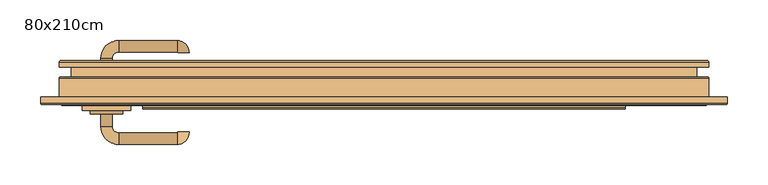
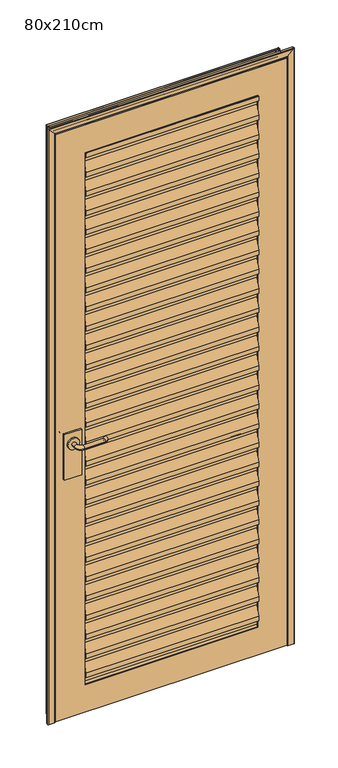
"""IFC4 building model written with IfcOpenShell, lengths in millimetres: door geometry, Porta de Abrir Metálica Veneziana : 80x210cm."""

from ifc_helpers import new_model, si_unit, point, frame, frame_2d, origin, place, context, project, spatial, polyline, circle_curve, ellipse_curve, trimmed, segment, composite_curve, outline, extrude, source, transform, mapped, element, save
from ifc_brep_helpers import plane_surface, cylinder_surface, revolved_surface, advanced_brep


def door_80x210cm_8dccb80e(model_context):
    return source(origin(), model_context, "Body", "SolidModel", [
        extrude(outline(polyline([(-88.9, 180.8599451), (-88.9, 160.8599451), (-91.1571429, 152.9599451), (-92.1971586, 152.9599451), (-89.9, 161.0), (-89.9, 179.8599451), (-99.9, 179.8599451), (-99.9, 196.0), (-89.9, 231.0), (-89.9, 249.8599451), (-99.9, 249.8599451), (-99.9, 266.0), (-89.9, 301.0), (-89.9, 319.8599451), (-99.9, 319.8599451), (-99.9, 336.0), (-89.9, 371.0), (-89.9, 389.8599451), (-99.9, 389.8599451), (-99.9, 406.0), (-89.9, 441.0), (-89.9, 459.8599451), (-99.9, 459.8599451), (-99.9, 476.0), (-89.9, 511.0), (-89.9, 529.8599451), (-99.9, 529.8599451), (-99.9, 546.0), (-89.9, 581.0), (-89.9, 599.8599451), (-99.9, 599.8599451), (-99.9, 616.0), (-89.9, 651.0), (-89.9, 669.8599451), (-99.9, 669.8599451), (-99.9, 686.0), (-89.9, 721.0), (-89.9, 739.8599451), (-99.9, 739.8599451), (-99.9, 756.0), (-89.9, 791.0), (-89.9, 809.8599451), (-99.9, 809.8599451), (-99.9, 826.0), (-89.9, 861.0), (-89.9, 879.8599451), (-99.9, 879.8599451), (-99.9, 896.0), (-89.9, 931.0), (-89.9, 949.8599451), (-99.9, 949.8599451), (-99.9, 966.0), (-89.9, 1001.0), (-89.9, 1019.8599451), (-99.9, 1019.8599451), (-99.9, 1036.0), (-89.9, 1071.0), (-89.9, 1089.8599451), (-99.9, 1089.8599451), (-99.9, 1106.0), (-89.9, 1141.0), (-89.9, 1159.8599451), (-99.9, 1159.8599451), (-99.9, 1176.0), (-89.9, 1211.0), (-89.9, 1229.8599451), (-99.9, 1229.8599451), (-99.9, 1246.0), (-89.9, 1281.0), (-89.9, 1299.8599451), (-99.9, 1299.8599451), (-99.9, 1316.0), (-89.9, 1351.0), (-89.9, 1369.8599451), (-99.9, 1369.8599451), (-99.9, 1386.0), (-89.9, 1421.0), (-89.9, 1439.8599451), (-99.9, 1439.8599451), (-99.9, 1456.0), (-89.9, 1491.0), (-89.9, 1509.8599451), (-99.9, 1509.8599451), (-99.9, 1526.0), (-89.9, 1561.0), (-89.9, 1579.8599451), (-99.9, 1579.8599451), (-99.9, 1596.0), (-89.9, 1631.0), (-89.9, 1649.8599451), (-99.9, 1649.8599451), (-99.9, 1666.0), (-89.9, 1701.0), (-89.9, 1719.8599451), (-99.9, 1719.8599451), (-99.9, 1736.0), (-89.9, 1771.0), (-89.9, 1789.8599451), (-99.9, 1789.8599451), (-99.9, 1806.0), (-89.9, 1841.0), (-89.9, 1859.8599451), (-99.9, 1859.8599451), (-99.9, 1876.0), (-89.9, 1911.0), (-89.9, 1929.8599451), (-99.9, 1929.8599451), (-99.9, 1946.0), (-89.9, 1981.0), (-89.9, 1999.8599451), (-99.9, 1999.8599451), (-99.9, 2016.0), (-89.9, 2051.0), (-89.9, 2069.8599451), (-99.9, 2069.8599451), (-99.9, 2086.0), (-98.9, 2085.8599451), (-98.9, 2070.8599451), (-88.9, 2070.8599451), (-88.9, 2050.8599451), (-98.9, 2015.8599451), (-98.9, 2000.8599451), (-88.9, 2000.8599451), (-88.9, 1980.8599451), (-98.9, 1945.8599451), (-98.9, 1930.8599451), (-88.9, 1930.8599451), (-88.9, 1910.8599451), (-98.9, 1875.8599451), (-98.9, 1860.8599451), (-88.9, 1860.8599451), (-88.9, 1840.8599451), (-98.9, 1805.8599451), (-98.9, 1790.8599451), (-88.9, 1790.8599451), (-88.9, 1770.8599451), (-98.9, 1735.8599451), (-98.9, 1720.8599451), (-88.9, 1720.8599451), (-88.9, 1700.8599451), (-98.9, 1665.8599451), (-98.9, 1650.8599451), (-88.9, 1650.8599451), (-88.9, 1630.8599451), (-98.9, 1595.8599451), (-98.9, 1580.8599451), (-88.9, 1580.8599451), (-88.9, 1560.8599451), (-98.9, 1525.8599451), (-98.9, 1510.8599451), (-88.9, 1510.8599451), (-88.9, 1490.8599451), (-98.9, 1455.8599451), (-98.9, 1440.8599451), (-88.9, 1440.8599451), (-88.9, 1420.8599451), (-98.9, 1385.8599451), (-98.9, 1370.8599451), (-88.9, 1370.8599451), (-88.9, 1350.8599451), (-98.9, 1315.8599451), (-98.9, 1300.8599451), (-88.9, 1300.8599451), (-88.9, 1280.8599451), (-98.9, 1245.8599451), (-98.9, 1230.8599451), (-88.9, 1230.8599451), (-88.9, 1210.8599451), (-98.9, 1175.8599451), (-98.9, 1160.8599451), (-88.9, 1160.8599451), (-88.9, 1140.8599451), (-98.9, 1105.8599451), (-98.9, 1090.8599451), (-88.9, 1090.8599451), (-88.9, 1070.8599451), (-98.9, 1035.8599451), (-98.9, 1020.8599451), (-88.9, 1020.8599451), (-88.9, 1000.8599451), (-98.9, 965.8599451), (-98.9, 950.8599451), (-88.9, 950.8599451), (-88.9, 930.8599451), (-98.9, 895.8599451), (-98.9, 880.8599451), (-88.9, 880.8599451), (-88.9, 860.8599451), (-98.9, 825.8599451), (-98.9, 810.8599451), (-88.9, 810.8599451), (-88.9, 790.8599451), (-98.9, 755.8599451), (-98.9, 740.8599451), (-88.9, 740.8599451), (-88.9, 720.8599451), (-98.9, 685.8599451), (-98.9, 670.8599451), (-88.9, 670.8599451), (-88.9, 650.8599451), (-98.9, 615.8599451), (-98.9, 600.8599451), (-88.9, 600.8599451), (-88.9, 580.8599451), (-98.9, 545.8599451), (-98.9, 530.8599451), (-88.9, 530.8599451), (-88.9, 510.8599451), (-98.9, 475.8599451), (-98.9, 460.8599451), (-88.9, 460.8599451), (-88.9, 440.8599451), (-98.9, 405.8599451), (-98.9, 390.8599451), (-88.9, 390.8599451), (-88.9, 370.8599451), (-98.9, 335.8599451), (-98.9, 320.8599451), (-88.9, 320.8599451), (-88.9, 300.8599451), (-98.9, 265.8599451), (-98.9, 250.8599451), (-88.9, 250.8599451), (-88.9, 230.8599451), (-98.9, 195.8599451), (-98.9, 180.8599451), (-88.9, 180.8599451)])), frame((-397.0, 0.0, 0.0), z_axis=(1.0, 0.0, 0.0), x_axis=(0.0, 1.0, 0.0)), (0.0, 0.0, 1.0), 594.0),
        extrude(outline(composite_curve([segment(trimmed(circle_curve(frame_2d((1050.0, -442.0)), 20.0), [point((1050.0, -462.0))], [point((1050.0, -422.0))], False, "CARTESIAN"), True, "CONTINUOUS"), segment(trimmed(circle_curve(frame_2d((1050.0, -442.0)), 20.0), [point((1050.0, -422.0))], [point((1050.0, -462.0))], False, "CARTESIAN"), True, "CONTINUOUS")], self_intersect=False)), frame((0.0, -57.6, 0.0), z_axis=(0.0, 1.0, 0.0), x_axis=(0.0, 0.0, 1.0)), (0.0, 0.0, 1.0), 4.5929895),
        advanced_brep(
        [(-435.0, -53.0070105, 1050.0), (-449.0, -53.0070105, 1050.0), (-435.0, -37.6, 1050.0), (-449.0, -37.6, 1050.0), (-427.0, -15.6, 1050.0), (-427.0, -29.6, 1050.0), (-355.0, -29.6, 1050.0), (-355.0, -15.6, 1050.0), (-354.0, -30.6, 1050.0), (-340.0, -30.6, 1050.0)],
        [
            (0, 1, circle_curve(frame((-442.0, -53.0070105, 1050.0), z_axis=(0.0, -1.0, 0.0), x_axis=(-1.0, 0.0, 0.0)), 7.0)),
            (1, 0, circle_curve(frame((-442.0, -53.0070105, 1050.0), z_axis=(0.0, -1.0, 0.0), x_axis=(-1.0, 0.0, 0.0)), 7.0)),
            (0, 2),
            (2, 3, circle_curve(frame((-442.0, -37.6, 1050.0), z_axis=(0.0, -1.0, 0.0), x_axis=(-1.0, 0.0, 0.0)), 7.0)),
            (3, 1),
            (3, 2, circle_curve(frame((-442.0, -37.6, 1050.0), z_axis=(0.0, -1.0, 0.0), x_axis=(-1.0, 0.0, 0.0)), 7.0)),
            (4, 3, circle_curve(frame((-427.0, -37.6, 1050.0), z_axis=(0.0, 0.0, 1.0), x_axis=(-1.0, 0.0, 0.0)), 22.0)),
            (2, 5, circle_curve(frame((-427.0, -37.6, 1050.0), z_axis=(0.0, 0.0, -1.0), x_axis=(-1.0, 0.0, 0.0)), 8.0)),
            (5, 4, circle_curve(frame((-427.0, -22.6, 1050.0), z_axis=(-1.0, 0.0, 0.0), x_axis=(0.0, 1.0, 0.0)), 7.0)),
            (4, 5, circle_curve(frame((-427.0, -22.6, 1050.0), z_axis=(-1.0, 0.0, 0.0), x_axis=(0.0, 1.0, 0.0)), 7.0)),
            (5, 6),
            (6, 7, circle_curve(frame((-355.0, -22.6, 1050.0), z_axis=(-1.0, 0.0, 0.0), x_axis=(0.0, 1.0, 0.0)), 7.0)),
            (7, 4),
            (7, 6, circle_curve(frame((-355.0, -22.6, 1050.0), z_axis=(-1.0, 0.0, 0.0), x_axis=(0.0, 1.0, 0.0)), 7.0)),
            (8, 9, circle_curve(frame((-347.0, -30.6, 1050.0), z_axis=(0.0, -1.0, 0.0), x_axis=(1.0, 0.0, 0.0)), 7.0)),
            (9, 8, circle_curve(frame((-347.0, -30.6, 1050.0), z_axis=(0.0, -1.0, 0.0), x_axis=(1.0, 0.0, 0.0)), 7.0)),
            (9, 7, circle_curve(frame((-355.0, -30.6, 1050.0), z_axis=(0.0, 0.0, 1.0), x_axis=(0.0, 1.0, 0.0)), 15.0)),
            (6, 8, circle_curve(frame((-355.0, -30.6, 1050.0), z_axis=(0.0, 0.0, -1.0), x_axis=(0.0, 1.0, 0.0)), 1.0)),
        ],
        [
            plane_surface(frame((-442.0, -53.0070105, 1050.0), z_axis=(0.0, -1.0, 0.0), x_axis=(0.0, 0.0, 1.0))),
            cylinder_surface(frame((-442.0, -53.0070105, 1050.0), z_axis=(0.0, -1.0, 0.0), x_axis=(-1.0, 0.0, 0.0)), 7.0),
            revolved_surface(trimmed(ellipse_curve(frame((-442.0, -37.6, 1050.0), z_axis=(0.0, -1.0, 0.0), x_axis=(-1.0, 0.0, 0.0)), 7.0, 7.0), [point((-435.0, -37.6, 1050.0))], [point((-449.0, -37.6, 1050.0))], True, "CARTESIAN"), (-427.0, -37.6, 1050.0), (0.0, 0.0, -1.0)),
            revolved_surface(trimmed(ellipse_curve(frame((-442.0, -37.6, 1050.0), z_axis=(0.0, -1.0, 0.0), x_axis=(-1.0, 0.0, 0.0)), 7.0, 7.0), [point((-449.0, -37.6, 1050.0))], [point((-435.0, -37.6, 1050.0))], True, "CARTESIAN"), (-427.0, -37.6, 1050.0), (0.0, 0.0, -1.0)),
            cylinder_surface(frame((-427.0, -22.6, 1050.0), z_axis=(-1.0, 0.0, 0.0), x_axis=(0.0, 1.0, 0.0)), 7.0),
            plane_surface(frame((-347.0, -30.6, 1050.0), z_axis=(0.0, -1.0, 0.0), x_axis=(0.0, 0.0, 1.0))),
            revolved_surface(trimmed(ellipse_curve(frame((-355.0, -22.6, 1050.0), z_axis=(-1.0, 0.0, 0.0), x_axis=(0.0, 1.0, 0.0)), 7.0, 7.0), [point((-355.0, -29.6, 1050.0))], [point((-355.0, -15.6, 1050.0))], True, "CARTESIAN"), (-355.0, -30.6, 1050.0), (0.0, 0.0, -1.0)),
            revolved_surface(trimmed(ellipse_curve(frame((-355.0, -22.6, 1050.0), z_axis=(-1.0, 0.0, 0.0), x_axis=(0.0, 1.0, 0.0)), 7.0, 7.0), [point((-355.0, -15.6, 1050.0))], [point((-355.0, -29.6, 1050.0))], True, "CARTESIAN"), (-355.0, -30.6, 1050.0), (0.0, 0.0, -1.0)),
        ],
        [
            (0, [[1, 2]]),
            (1, [[-1, 3, 4, 5]]),
            (1, [[-2, -5, 6, -3]]),
            (2, [[7, -4, 8, 9]]),
            (3, [[-8, -6, -7, 10]]),
            (4, [[-9, 11, 12, 13]]),
            (4, [[-10, -13, 14, -11]]),
            (5, [[15, 16]]),
            (6, [[17, -12, 18, -16]]),
            (7, [[-18, -14, -17, -15]]),
        ],
    ),
        extrude(outline(polyline([(-412.0, -63.6), (-472.0, -63.6), (-472.0, -57.6), (-412.0, -57.6), (-412.0, -63.6)])), frame((0.0, 0.0, 925.0), z_axis=(0.0, 0.0, 1.0), x_axis=(1.0, 0.0, 0.0)), (0.0, 0.0, 1.0), 165.0),
        extrude(outline(composite_curve([segment(trimmed(circle_curve(frame_2d((1050.0, -442.0)), 20.0), [point((1050.0, -462.0))], [point((1050.0, -422.0))], False, "CARTESIAN"), True, "CONTINUOUS"), segment(trimmed(circle_curve(frame_2d((1050.0, -442.0)), 20.0), [point((1050.0, -422.0))], [point((1050.0, -462.0))], False, "CARTESIAN"), True, "CONTINUOUS")], self_intersect=False)), frame((0.0, -106.1929895, 0.0), z_axis=(0.0, 1.0, 0.0), x_axis=(0.0, 0.0, 1.0)), (0.0, 0.0, 1.0), 4.5929895),
        advanced_brep(
        [(-435.0, -106.1929895, 1050.0), (-449.0, -106.1929895, 1050.0), (-449.0, -121.6, 1050.0), (-435.0, -121.6, 1050.0), (-427.0, -143.6, 1050.0), (-427.0, -129.6, 1050.0), (-355.0, -143.6, 1050.0), (-355.0, -129.6, 1050.0), (-354.0, -128.6, 1050.0), (-340.0, -128.6, 1050.0)],
        [
            (0, 1, circle_curve(frame((-442.0, -106.1929895, 1050.0), z_axis=(0.0, 1.0, 0.0), x_axis=(-1.0, 0.0, 0.0)), 7.0)),
            (1, 0, circle_curve(frame((-442.0, -106.1929895, 1050.0), z_axis=(0.0, 1.0, 0.0), x_axis=(-1.0, 0.0, 0.0)), 7.0)),
            (1, 2),
            (2, 3, circle_curve(frame((-442.0, -121.6, 1050.0), z_axis=(0.0, 1.0, 0.0), x_axis=(-1.0, 0.0, 0.0)), 7.0)),
            (3, 0),
            (3, 2, circle_curve(frame((-442.0, -121.6, 1050.0), z_axis=(0.0, 1.0, 0.0), x_axis=(-1.0, 0.0, 0.0)), 7.0)),
            (4, 5, circle_curve(frame((-427.0, -136.6, 1050.0), z_axis=(-1.0, 0.0, 0.0), x_axis=(0.0, -1.0, 0.0)), 7.0)),
            (5, 3, circle_curve(frame((-427.0, -121.6, 1050.0), z_axis=(0.0, 0.0, -1.0), x_axis=(-1.0, 0.0, 0.0)), 8.0)),
            (2, 4, circle_curve(frame((-427.0, -121.6, 1050.0), z_axis=(0.0, 0.0, 1.0), x_axis=(-1.0, 0.0, 0.0)), 22.0)),
            (5, 4, circle_curve(frame((-427.0, -136.6, 1050.0), z_axis=(-1.0, 0.0, 0.0), x_axis=(0.0, -1.0, 0.0)), 7.0)),
            (4, 6),
            (6, 7, circle_curve(frame((-355.0, -136.6, 1050.0), z_axis=(-1.0, 0.0, 0.0), x_axis=(0.0, -1.0, 0.0)), 7.0)),
            (7, 5),
            (7, 6, circle_curve(frame((-355.0, -136.6, 1050.0), z_axis=(-1.0, 0.0, 0.0), x_axis=(0.0, -1.0, 0.0)), 7.0)),
            (8, 9, circle_curve(frame((-347.0, -128.6, 1050.0), z_axis=(0.0, 1.0, 0.0), x_axis=(1.0, 0.0, 0.0)), 7.0)),
            (9, 8, circle_curve(frame((-347.0, -128.6, 1050.0), z_axis=(0.0, 1.0, 0.0), x_axis=(1.0, 0.0, 0.0)), 7.0)),
            (8, 7, circle_curve(frame((-355.0, -128.6, 1050.0), z_axis=(0.0, 0.0, -1.0), x_axis=(0.0, -1.0, 0.0)), 1.0)),
            (6, 9, circle_curve(frame((-355.0, -128.6, 1050.0), z_axis=(0.0, 0.0, 1.0), x_axis=(0.0, -1.0, 0.0)), 15.0)),
        ],
        [
            plane_surface(frame((-442.0, -106.1929895, 1050.0), z_axis=(0.0, 1.0, 0.0), x_axis=(0.0, 0.0, 1.0))),
            cylinder_surface(frame((-442.0, -106.1929895, 1050.0), z_axis=(0.0, 1.0, 0.0), x_axis=(-1.0, 0.0, 0.0)), 7.0),
            revolved_surface(trimmed(ellipse_curve(frame((-442.0, -121.6, 1050.0), z_axis=(0.0, -1.0, 0.0), x_axis=(-1.0, 0.0, 0.0)), 7.0, 7.0), [point((-435.0, -121.6, 1050.0))], [point((-449.0, -121.6, 1050.0))], True, "CARTESIAN"), (-427.0, -121.6, 1050.0), (0.0, 0.0, -1.0)),
            revolved_surface(trimmed(ellipse_curve(frame((-442.0, -121.6, 1050.0), z_axis=(0.0, -1.0, 0.0), x_axis=(-1.0, 0.0, 0.0)), 7.0, 7.0), [point((-449.0, -121.6, 1050.0))], [point((-435.0, -121.6, 1050.0))], True, "CARTESIAN"), (-427.0, -121.6, 1050.0), (0.0, 0.0, -1.0)),
            cylinder_surface(frame((-427.0, -136.6, 1050.0), z_axis=(-1.0, 0.0, 0.0), x_axis=(0.0, -1.0, 0.0)), 7.0),
            plane_surface(frame((-347.0, -128.6, 1050.0), z_axis=(0.0, 1.0, 0.0), x_axis=(0.0, 0.0, 1.0))),
            revolved_surface(trimmed(ellipse_curve(frame((-355.0, -136.6, 1050.0), z_axis=(1.0, 0.0, 0.0), x_axis=(0.0, -1.0, 0.0)), 7.0, 7.0), [point((-355.0, -129.6, 1050.0))], [point((-355.0, -143.6, 1050.0))], True, "CARTESIAN"), (-355.0, -128.6, 1050.0), (0.0, 0.0, -1.0)),
            revolved_surface(trimmed(ellipse_curve(frame((-355.0, -136.6, 1050.0), z_axis=(1.0, 0.0, 0.0), x_axis=(0.0, -1.0, 0.0)), 7.0, 7.0), [point((-355.0, -143.6, 1050.0))], [point((-355.0, -129.6, 1050.0))], True, "CARTESIAN"), (-355.0, -128.6, 1050.0), (0.0, 0.0, -1.0)),
        ],
        [
            (0, [[1, 2]]),
            (1, [[3, 4, 5, -2]]),
            (1, [[-5, 6, -3, -1]]),
            (2, [[7, 8, -4, 9]]),
            (3, [[10, -9, -6, -8]]),
            (4, [[11, 12, 13, -7]]),
            (4, [[-13, 14, -11, -10]]),
            (5, [[15, 16]]),
            (6, [[-15, 17, -12, 18]]),
            (7, [[-16, -18, -14, -17]]),
        ],
    ),
        extrude(outline(polyline([(-412.0, -95.6), (-412.0, -101.6), (-472.0, -101.6), (-472.0, -95.6), (-412.0, -95.6)])), frame((0.0, 0.0, 925.0), z_axis=(0.0, 0.0, 1.0), x_axis=(1.0, 0.0, 0.0)), (0.0, 0.0, 1.0), 165.0),
        extrude(outline(polyline([(2186.0, -497.0), (53.0, -497.0), (53.0, 297.0), (2186.0, 297.0), (2186.0, -497.0)]), holes=[polyline([(2086.0, -397.0), (2086.0, 197.0), (153.0, 197.0), (153.0, -397.0), (2086.0, -397.0)])]), frame((0.0, -95.6, 0.0), z_axis=(0.0, 1.0, 0.0), x_axis=(0.0, 0.0, 1.0)), (0.0, 0.0, 1.0), 32.0),
        advanced_brep(
        [(-485.5, -40.6, 50.0), (-484.0, -42.1, 50.0), (-484.0, -60.1, 50.0), (-485.5, -61.6, 50.0), (-498.55, -61.6, 50.0), (-499.05, -62.1, 50.0), (-499.05, -93.1, 50.0), (-500.55, -94.6, 50.0), (-521.55, -94.6, 50.0), (-523.05, -93.1, 50.0), (-523.05, -85.6, 50.0), (-522.05, -85.6, 50.0), (-522.05, -93.1, 50.0), (-521.55, -93.6, 50.0), (-500.55, -93.6, 50.0), (-500.05, -93.1, 50.0), (-500.05, -62.1, 50.0), (-498.55, -60.6, 50.0), (-485.5, -60.6, 50.0), (-485.0, -60.1, 50.0), (-485.0, -42.1, 50.0), (-485.5, -41.6, 50.0), (-498.5, -41.6, 50.0), (-499.0, -42.1, 50.0), (-499.0, -48.6, 50.0), (-500.0, -48.6, 50.0), (-500.0, -42.1, 50.0), (-498.5, -40.6, 50.0), (-498.5, -40.6, 2188.5), (-485.5, -40.6, 2175.5), (-500.0, -42.1, 2190.0), (-500.0, -48.6, 2190.0), (-499.0, -48.6, 2189.0), (-499.0, -42.1, 2189.0), (-498.5, -41.6, 2188.5), (-485.5, -41.6, 2175.5), (-485.0, -42.1, 2175.0), (-485.0, -60.1, 2175.0), (-485.5, -60.6, 2175.5), (-498.55, -60.6, 2188.55), (-500.05, -62.1, 2190.05), (-500.05, -93.1, 2190.05), (-500.55, -93.6, 2190.55), (-521.55, -93.6, 2211.55), (-522.05, -93.1, 2212.05), (-522.05, -85.6, 2212.05), (-523.05, -85.6, 2213.05), (-523.05, -93.1, 2213.05), (-521.55, -94.6, 2211.55), (-500.55, -94.6, 2190.55), (-499.05, -93.1, 2189.05), (-499.05, -62.1, 2189.05), (-498.55, -61.6, 2188.55), (-485.5, -61.6, 2175.5), (-484.0, -60.1, 2174.0), (-484.0, -42.1, 2174.0), (285.5, -40.6, 50.0), (298.5, -40.6, 50.0), (300.0, -42.1, 50.0), (300.0, -48.6, 50.0), (299.0, -48.6, 50.0), (299.0, -42.1, 50.0), (298.5, -41.6, 50.0), (285.5, -41.6, 50.0), (285.0, -42.1, 50.0), (285.0, -60.1, 50.0), (285.5, -60.6, 50.0), (298.55, -60.6, 50.0), (300.05, -62.1, 50.0), (300.05, -93.1, 50.0), (300.55, -93.6, 50.0), (321.55, -93.6, 50.0), (322.05, -93.1, 50.0), (322.05, -85.6, 50.0), (323.05, -85.6, 50.0), (323.05, -93.1, 50.0), (321.55, -94.6, 50.0), (300.55, -94.6, 50.0), (299.05, -93.1, 50.0), (299.05, -62.1, 50.0), (298.55, -61.6, 50.0), (285.5, -61.6, 50.0), (284.0, -60.1, 50.0), (284.0, -42.1, 50.0), (285.5, -40.6, 2175.5), (284.0, -42.1, 2174.0), (284.0, -60.1, 2174.0), (285.5, -61.6, 2175.5), (298.55, -61.6, 2188.55), (299.05, -62.1, 2189.05), (299.05, -93.1, 2189.05), (300.55, -94.6, 2190.55), (321.55, -94.6, 2211.55), (323.05, -93.1, 2213.05), (323.05, -85.6, 2213.05), (322.05, -85.6, 2212.05), (322.05, -93.1, 2212.05), (321.55, -93.6, 2211.55), (300.55, -93.6, 2190.55), (300.05, -93.1, 2190.05), (300.05, -62.1, 2190.05), (298.55, -60.6, 2188.55), (285.5, -60.6, 2175.5), (285.0, -60.1, 2175.0), (285.0, -42.1, 2175.0), (285.5, -41.6, 2175.5), (298.5, -41.6, 2188.5), (299.0, -42.1, 2189.0), (299.0, -48.6, 2189.0), (300.0, -48.6, 2190.0), (300.0, -42.1, 2190.0), (298.5, -40.6, 2188.5)],
        [
            (0, 1, circle_curve(frame((-485.5, -42.1, 50.0), z_axis=(0.0, 0.0, -1.0), x_axis=(1.0, 0.0, 0.0)), 1.5)),
            (1, 2),
            (2, 3, circle_curve(frame((-485.5, -60.1, 50.0), z_axis=(0.0, 0.0, -1.0), x_axis=(1.0, 0.0, 0.0)), 1.5)),
            (3, 4),
            (4, 5, circle_curve(frame((-498.55, -62.1, 50.0), z_axis=(0.0, 0.0, 1.0), x_axis=(1.0, 0.0, 0.0)), 0.5)),
            (5, 6),
            (6, 7, circle_curve(frame((-500.55, -93.1, 50.0), z_axis=(0.0, 0.0, -1.0), x_axis=(1.0, 0.0, 0.0)), 1.5)),
            (7, 8),
            (8, 9, circle_curve(frame((-521.55, -93.1, 50.0), z_axis=(0.0, 0.0, -1.0), x_axis=(1.0, 0.0, 0.0)), 1.5)),
            (9, 10),
            (10, 11),
            (11, 12),
            (12, 13, circle_curve(frame((-521.55, -93.1, 50.0), z_axis=(0.0, 0.0, 1.0), x_axis=(1.0, 0.0, 0.0)), 0.5)),
            (13, 14),
            (14, 15, circle_curve(frame((-500.55, -93.1, 50.0), z_axis=(0.0, 0.0, 1.0), x_axis=(1.0, 0.0, 0.0)), 0.5)),
            (15, 16),
            (16, 17, circle_curve(frame((-498.55, -62.1, 50.0), z_axis=(0.0, 0.0, -1.0), x_axis=(1.0, 0.0, 0.0)), 1.5)),
            (17, 18),
            (18, 19, circle_curve(frame((-485.5, -60.1, 50.0), z_axis=(0.0, 0.0, 1.0), x_axis=(1.0, 0.0, 0.0)), 0.5)),
            (19, 20),
            (20, 21, circle_curve(frame((-485.5, -42.1, 50.0), z_axis=(0.0, 0.0, 1.0), x_axis=(1.0, 0.0, 0.0)), 0.5)),
            (21, 22),
            (22, 23, circle_curve(frame((-498.5, -42.1, 50.0), z_axis=(0.0, 0.0, 1.0), x_axis=(1.0, 0.0, 0.0)), 0.5)),
            (23, 24),
            (24, 25),
            (25, 26),
            (26, 27, circle_curve(frame((-498.5, -42.1, 50.0), z_axis=(0.0, 0.0, -1.0), x_axis=(1.0, 0.0, 0.0)), 1.5)),
            (27, 0),
            (27, 28),
            (28, 29),
            (29, 0),
            (26, 30),
            (30, 28, ellipse_curve(frame((-498.5, -42.1, 2188.5), z_axis=(-0.7071067811865475, 0.0, -0.7071067811865475), x_axis=(0.7071067811865474, 0.0, -0.7071067811865476)), 2.1213203, 1.5)),
            (25, 31),
            (31, 30),
            (24, 32),
            (32, 31),
            (23, 33),
            (33, 32),
            (22, 34),
            (34, 33, ellipse_curve(frame((-498.5, -42.1, 2188.5), z_axis=(0.7071067811865475, 0.0, 0.7071067811865475), x_axis=(-0.7071067811865474, 0.0, 0.7071067811865476)), 0.7071068, 0.5)),
            (21, 35),
            (35, 34),
            (20, 36),
            (36, 35, ellipse_curve(frame((-485.5, -42.1, 2175.5), z_axis=(0.7071067811865475, 0.0, 0.7071067811865475), x_axis=(-0.7071067811865474, 0.0, 0.7071067811865476)), 0.7071068, 0.5)),
            (19, 37),
            (37, 36),
            (18, 38),
            (38, 37, ellipse_curve(frame((-485.5, -60.1, 2175.5), z_axis=(0.7071067811865475, 0.0, 0.7071067811865475), x_axis=(-0.7071067811865474, 0.0, 0.7071067811865476)), 0.7071068, 0.5)),
            (17, 39),
            (39, 38),
            (16, 40),
            (40, 39, ellipse_curve(frame((-498.55, -62.1, 2188.55), z_axis=(-0.7071067811865475, 0.0, -0.7071067811865475), x_axis=(0.7071067811865474, 0.0, -0.7071067811865476)), 2.1213203, 1.5)),
            (15, 41),
            (41, 40),
            (14, 42),
            (42, 41, ellipse_curve(frame((-500.55, -93.1, 2190.55), z_axis=(0.7071067811865475, 0.0, 0.7071067811865475), x_axis=(-0.7071067811865474, 0.0, 0.7071067811865476)), 0.7071068, 0.5)),
            (13, 43),
            (43, 42),
            (12, 44),
            (44, 43, ellipse_curve(frame((-521.55, -93.1, 2211.55), z_axis=(0.7071067811865475, 0.0, 0.7071067811865475), x_axis=(-0.7071067811865474, 0.0, 0.7071067811865476)), 0.7071068, 0.5)),
            (11, 45),
            (45, 44),
            (10, 46),
            (46, 45),
            (9, 47),
            (47, 46),
            (8, 48),
            (48, 47, ellipse_curve(frame((-521.55, -93.1, 2211.55), z_axis=(-0.7071067811865475, 0.0, -0.7071067811865475), x_axis=(0.7071067811865474, 0.0, -0.7071067811865476)), 2.1213203, 1.5)),
            (7, 49),
            (49, 48),
            (6, 50),
            (50, 49, ellipse_curve(frame((-500.55, -93.1, 2190.55), z_axis=(-0.7071067811865475, 0.0, -0.7071067811865475), x_axis=(0.7071067811865474, 0.0, -0.7071067811865476)), 2.1213203, 1.5)),
            (5, 51),
            (51, 50),
            (4, 52),
            (52, 51, ellipse_curve(frame((-498.55, -62.1, 2188.55), z_axis=(0.7071067811865475, 0.0, 0.7071067811865475), x_axis=(-0.7071067811865474, 0.0, 0.7071067811865476)), 0.7071068, 0.5)),
            (3, 53),
            (53, 52),
            (2, 54),
            (54, 53, ellipse_curve(frame((-485.5, -60.1, 2175.5), z_axis=(-0.7071067811865475, 0.0, -0.7071067811865475), x_axis=(0.7071067811865474, 0.0, -0.7071067811865476)), 2.1213203, 1.5)),
            (1, 55),
            (55, 54),
            (29, 55, ellipse_curve(frame((-485.5, -42.1, 2175.5), z_axis=(-0.7071067811865475, 0.0, -0.7071067811865475), x_axis=(0.7071067811865474, 0.0, -0.7071067811865476)), 2.1213203, 1.5)),
            (56, 57),
            (57, 58, circle_curve(frame((298.5, -42.1, 50.0), z_axis=(0.0, 0.0, -1.0), x_axis=(-1.0, 0.0, 0.0)), 1.5)),
            (58, 59),
            (59, 60),
            (60, 61),
            (61, 62, circle_curve(frame((298.5, -42.1, 50.0), z_axis=(0.0, 0.0, 1.0), x_axis=(-1.0, 0.0, 0.0)), 0.5)),
            (62, 63),
            (63, 64, circle_curve(frame((285.5, -42.1, 50.0), z_axis=(0.0, 0.0, 1.0), x_axis=(-1.0, 0.0, 0.0)), 0.5)),
            (64, 65),
            (65, 66, circle_curve(frame((285.5, -60.1, 50.0), z_axis=(0.0, 0.0, 1.0), x_axis=(-1.0, 0.0, 0.0)), 0.5)),
            (66, 67),
            (67, 68, circle_curve(frame((298.55, -62.1, 50.0), z_axis=(0.0, 0.0, -1.0), x_axis=(-1.0, 0.0, 0.0)), 1.5)),
            (68, 69),
            (69, 70, circle_curve(frame((300.55, -93.1, 50.0), z_axis=(0.0, 0.0, 1.0), x_axis=(-1.0, 0.0, 0.0)), 0.5)),
            (70, 71),
            (71, 72, circle_curve(frame((321.55, -93.1, 50.0), z_axis=(0.0, 0.0, 1.0), x_axis=(-1.0, 0.0, 0.0)), 0.5)),
            (72, 73),
            (73, 74),
            (74, 75),
            (75, 76, circle_curve(frame((321.55, -93.1, 50.0), z_axis=(0.0, 0.0, -1.0), x_axis=(-1.0, 0.0, 0.0)), 1.5)),
            (76, 77),
            (77, 78, circle_curve(frame((300.55, -93.1, 50.0), z_axis=(0.0, 0.0, -1.0), x_axis=(-1.0, 0.0, 0.0)), 1.5)),
            (78, 79),
            (79, 80, circle_curve(frame((298.55, -62.1, 50.0), z_axis=(0.0, 0.0, 1.0), x_axis=(-1.0, 0.0, 0.0)), 0.5)),
            (80, 81),
            (81, 82, circle_curve(frame((285.5, -60.1, 50.0), z_axis=(0.0, 0.0, -1.0), x_axis=(-1.0, 0.0, 0.0)), 1.5)),
            (82, 83),
            (83, 56, circle_curve(frame((285.5, -42.1, 50.0), z_axis=(0.0, 0.0, -1.0), x_axis=(-1.0, 0.0, 0.0)), 1.5)),
            (84, 56),
            (83, 85),
            (85, 84, ellipse_curve(frame((285.5, -42.1, 2175.5), z_axis=(0.7071067811865475, 0.0, -0.7071067811865475), x_axis=(0.7071067811865474, 0.0, 0.7071067811865476)), 2.1213203, 1.5)),
            (82, 86),
            (86, 85),
            (81, 87),
            (87, 86, ellipse_curve(frame((285.5, -60.1, 2175.5), z_axis=(0.7071067811865475, 0.0, -0.7071067811865475), x_axis=(0.7071067811865474, 0.0, 0.7071067811865476)), 2.1213203, 1.5)),
            (80, 88),
            (88, 87),
            (79, 89),
            (89, 88, ellipse_curve(frame((298.55, -62.1, 2188.55), z_axis=(-0.7071067811865475, 0.0, 0.7071067811865475), x_axis=(-0.7071067811865474, 0.0, -0.7071067811865476)), 0.7071068, 0.5)),
            (78, 90),
            (90, 89),
            (77, 91),
            (91, 90, ellipse_curve(frame((300.55, -93.1, 2190.55), z_axis=(0.7071067811865475, 0.0, -0.7071067811865475), x_axis=(0.7071067811865474, 0.0, 0.7071067811865476)), 2.1213203, 1.5)),
            (76, 92),
            (92, 91),
            (75, 93),
            (93, 92, ellipse_curve(frame((321.55, -93.1, 2211.55), z_axis=(0.7071067811865475, 0.0, -0.7071067811865475), x_axis=(0.7071067811865474, 0.0, 0.7071067811865476)), 2.1213203, 1.5)),
            (74, 94),
            (94, 93),
            (73, 95),
            (95, 94),
            (72, 96),
            (96, 95),
            (71, 97),
            (97, 96, ellipse_curve(frame((321.55, -93.1, 2211.55), z_axis=(-0.7071067811865475, 0.0, 0.7071067811865475), x_axis=(-0.7071067811865474, 0.0, -0.7071067811865476)), 0.7071068, 0.5)),
            (70, 98),
            (98, 97),
            (69, 99),
            (99, 98, ellipse_curve(frame((300.55, -93.1, 2190.55), z_axis=(-0.7071067811865475, 0.0, 0.7071067811865475), x_axis=(-0.7071067811865474, 0.0, -0.7071067811865476)), 0.7071068, 0.5)),
            (68, 100),
            (100, 99),
            (67, 101),
            (101, 100, ellipse_curve(frame((298.55, -62.1, 2188.55), z_axis=(0.7071067811865475, 0.0, -0.7071067811865475), x_axis=(0.7071067811865474, 0.0, 0.7071067811865476)), 2.1213203, 1.5)),
            (66, 102),
            (102, 101),
            (65, 103),
            (103, 102, ellipse_curve(frame((285.5, -60.1, 2175.5), z_axis=(-0.7071067811865475, 0.0, 0.7071067811865475), x_axis=(-0.7071067811865474, 0.0, -0.7071067811865476)), 0.7071068, 0.5)),
            (64, 104),
            (104, 103),
            (63, 105),
            (105, 104, ellipse_curve(frame((285.5, -42.1, 2175.5), z_axis=(-0.7071067811865475, 0.0, 0.7071067811865475), x_axis=(-0.7071067811865474, 0.0, -0.7071067811865476)), 0.7071068, 0.5)),
            (62, 106),
            (106, 105),
            (61, 107),
            (107, 106, ellipse_curve(frame((298.5, -42.1, 2188.5), z_axis=(-0.7071067811865475, 0.0, 0.7071067811865475), x_axis=(-0.7071067811865474, 0.0, -0.7071067811865476)), 0.7071068, 0.5)),
            (60, 108),
            (108, 107),
            (59, 109),
            (109, 108),
            (58, 110),
            (110, 109),
            (57, 111),
            (111, 110, ellipse_curve(frame((298.5, -42.1, 2188.5), z_axis=(0.7071067811865475, 0.0, -0.7071067811865475), x_axis=(0.7071067811865474, 0.0, 0.7071067811865476)), 2.1213203, 1.5)),
            (84, 111),
            (28, 111),
            (84, 29),
            (30, 110),
            (31, 109),
            (32, 108),
            (33, 107),
            (34, 106),
            (35, 105),
            (36, 104),
            (37, 103),
            (38, 102),
            (39, 101),
            (40, 100),
            (41, 99),
            (42, 98),
            (43, 97),
            (44, 96),
            (45, 95),
            (46, 94),
            (47, 93),
            (48, 92),
            (49, 91),
            (50, 90),
            (51, 89),
            (52, 88),
            (53, 87),
            (54, 86),
            (55, 85),
        ],
        [
            plane_surface(frame((-500.0, -38.3215694, 50.0), z_axis=(0.0, 0.0, -1.0), x_axis=(1.0, 0.0, 0.0))),
            plane_surface(frame((-485.5, -40.6, 50.0), z_axis=(0.0, 1.0, 0.0), x_axis=(0.0, 0.0, 1.0))),
            cylinder_surface(frame((-498.5, -42.1, 50.0), z_axis=(0.0, 0.0, -1.0), x_axis=(1.0, 0.0, 0.0)), 1.5),
            plane_surface(frame((-500.0, -42.1, 50.0), z_axis=(-1.0, 0.0, 0.0), x_axis=(0.0, 0.0, 1.0))),
            plane_surface(frame((-500.0, -48.6, 50.0), z_axis=(0.0, -1.0, 0.0), x_axis=(0.0, 0.0, 1.0))),
            plane_surface(frame((-499.0, -48.6, 50.0), z_axis=(1.0, 0.0, 0.0), x_axis=(0.0, 0.0, 1.0))),
            revolved_surface(polyline([(-498.0, -42.1, 2189.000000013303), (-498.0, -42.1, 50.0)]), (-498.5, -42.1, 50.0), (0.0, 0.0, 1.0)),
            plane_surface(frame((-498.5, -41.6, 50.0), z_axis=(0.0, -1.0, 0.0), x_axis=(0.0, 0.0, 1.0))),
            revolved_surface(polyline([(-485.0, -42.1, 2176.000000013303), (-485.0, -42.1, 50.0)]), (-485.5, -42.1, 50.0), (0.0, 0.0, 1.0)),
            plane_surface(frame((-485.0, -42.1, 50.0), z_axis=(-1.0, 0.0, 0.0), x_axis=(0.0, 0.0, 1.0))),
            revolved_surface(polyline([(-485.0, -60.1, 2176.000000013303), (-485.0, -60.1, 50.0)]), (-485.5, -60.1, 50.0), (0.0, 0.0, 1.0)),
            plane_surface(frame((-485.5, -60.6, 50.0), z_axis=(0.0, 1.0, 0.0), x_axis=(0.0, 0.0, 1.0))),
            cylinder_surface(frame((-498.55, -62.1, 50.0), z_axis=(0.0, 0.0, -1.0), x_axis=(1.0, 0.0, 0.0)), 1.5),
            plane_surface(frame((-500.05, -62.1, 50.0), z_axis=(-1.0, 0.0, 0.0), x_axis=(0.0, 0.0, 1.0))),
            revolved_surface(polyline([(-500.05, -93.1, 2191.0500000133034), (-500.05, -93.1, 50.0)]), (-500.55, -93.1, 50.0), (0.0, 0.0, 1.0)),
            plane_surface(frame((-500.55, -93.6, 50.0), z_axis=(0.0, 1.0, 0.0), x_axis=(0.0, 0.0, 1.0))),
            revolved_surface(polyline([(-521.05, -93.1, 2212.0500000133034), (-521.05, -93.1, 50.0)]), (-521.55, -93.1, 50.0), (0.0, 0.0, 1.0)),
            plane_surface(frame((-522.05, -93.1, 50.0), z_axis=(1.0, 0.0, 0.0), x_axis=(0.0, 0.0, 1.0))),
            plane_surface(frame((-522.05, -85.6, 50.0), z_axis=(0.0, 1.0, 0.0), x_axis=(0.0, 0.0, 1.0))),
            plane_surface(frame((-523.05, -85.6, 50.0), z_axis=(-1.0, 0.0, 0.0), x_axis=(0.0, 0.0, 1.0))),
            cylinder_surface(frame((-521.55, -93.1, 50.0), z_axis=(0.0, 0.0, -1.0), x_axis=(1.0, 0.0, 0.0)), 1.5),
            plane_surface(frame((-521.55, -94.6, 50.0), z_axis=(0.0, -1.0, 0.0), x_axis=(0.0, 0.0, 1.0))),
            cylinder_surface(frame((-500.55, -93.1, 50.0), z_axis=(0.0, 0.0, -1.0), x_axis=(1.0, 0.0, 0.0)), 1.5),
            plane_surface(frame((-499.05, -93.1, 50.0), z_axis=(1.0, 0.0, 0.0), x_axis=(0.0, 0.0, 1.0))),
            revolved_surface(polyline([(-498.05, -62.1, 2189.0500000133034), (-498.05, -62.1, 50.0)]), (-498.55, -62.1, 50.0), (0.0, 0.0, 1.0)),
            plane_surface(frame((-498.55, -61.6, 50.0), z_axis=(0.0, -1.0, 0.0), x_axis=(0.0, 0.0, 1.0))),
            cylinder_surface(frame((-485.5, -60.1, 50.0), z_axis=(0.0, 0.0, -1.0), x_axis=(1.0, 0.0, 0.0)), 1.5),
            plane_surface(frame((-484.0, -60.1, 50.0), z_axis=(1.0, 0.0, 0.0), x_axis=(0.0, 0.0, 1.0))),
            cylinder_surface(frame((-485.5, -42.1, 50.0), z_axis=(0.0, 0.0, -1.0), x_axis=(1.0, 0.0, 0.0)), 1.5),
            plane_surface(frame((300.0, -38.3215694, 50.0), z_axis=(0.0, 0.0, -1.0), x_axis=(-1.0, 0.0, 0.0))),
            cylinder_surface(frame((285.5, -42.1, 2190.0), z_axis=(0.0, 0.0, 1.0), x_axis=(-1.0, 0.0, 0.0)), 1.5),
            plane_surface(frame((284.0, -60.1, 2174.0), z_axis=(-1.0, 0.0, 0.0), x_axis=(0.0, 0.0, -1.0))),
            cylinder_surface(frame((285.5, -60.1, 2190.0), z_axis=(0.0, 0.0, 1.0), x_axis=(-1.0, 0.0, 0.0)), 1.5),
            plane_surface(frame((298.55, -61.6, 2188.55), z_axis=(0.0, -1.0, 0.0), x_axis=(0.0, 0.0, -1.0))),
            revolved_surface(polyline([(298.05, -62.1, 50.0), (298.05, -62.1, 2189.0500000133034)]), (298.55, -62.1, 2190.0), (0.0, 0.0, -1.0)),
            plane_surface(frame((299.05, -93.1, 2189.05), z_axis=(-1.0, 0.0, 0.0), x_axis=(0.0, 0.0, -1.0))),
            cylinder_surface(frame((300.55, -93.1, 2190.0), z_axis=(0.0, 0.0, 1.0), x_axis=(-1.0, 0.0, 0.0)), 1.5),
            plane_surface(frame((321.55, -94.6, 2211.55), z_axis=(0.0, -1.0, 0.0), x_axis=(0.0, 0.0, -1.0))),
            cylinder_surface(frame((321.55, -93.1, 2190.0), z_axis=(0.0, 0.0, 1.0), x_axis=(-1.0, 0.0, 0.0)), 1.5),
            plane_surface(frame((323.05, -85.6, 2213.05), z_axis=(1.0, 0.0, 0.0), x_axis=(0.0, 0.0, -1.0))),
            plane_surface(frame((322.05, -85.6, 2212.05), z_axis=(0.0, 1.0, 0.0), x_axis=(0.0, 0.0, -1.0))),
            plane_surface(frame((322.05, -93.1, 2212.05), z_axis=(-1.0, 0.0, 0.0), x_axis=(0.0, 0.0, -1.0))),
            revolved_surface(polyline([(321.05, -93.1, 50.0), (321.05, -93.1, 2212.0500000133034)]), (321.55, -93.1, 2190.0), (0.0, 0.0, -1.0)),
            plane_surface(frame((300.55, -93.6, 2190.55), z_axis=(0.0, 1.0, 0.0), x_axis=(0.0, 0.0, -1.0))),
            revolved_surface(polyline([(300.05, -93.1, 50.0), (300.05, -93.1, 2191.0500000133034)]), (300.55, -93.1, 2190.0), (0.0, 0.0, -1.0)),
            plane_surface(frame((300.05, -62.1, 2190.05), z_axis=(1.0, 0.0, 0.0), x_axis=(0.0, 0.0, -1.0))),
            cylinder_surface(frame((298.55, -62.1, 2190.0), z_axis=(0.0, 0.0, 1.0), x_axis=(-1.0, 0.0, 0.0)), 1.5),
            plane_surface(frame((285.5, -60.6, 2175.5), z_axis=(0.0, 1.0, 0.0), x_axis=(0.0, 0.0, -1.0))),
            revolved_surface(polyline([(285.0, -60.1, 50.0), (285.0, -60.1, 2176.000000013303)]), (285.5, -60.1, 2190.0), (0.0, 0.0, -1.0)),
            plane_surface(frame((285.0, -42.1, 2175.0), z_axis=(1.0, 0.0, 0.0), x_axis=(0.0, 0.0, -1.0))),
            revolved_surface(polyline([(285.0, -42.1, 50.0), (285.0, -42.1, 2176.000000013303)]), (285.5, -42.1, 2190.0), (0.0, 0.0, -1.0)),
            plane_surface(frame((298.5, -41.6, 2188.5), z_axis=(0.0, -1.0, 0.0), x_axis=(0.0, 0.0, -1.0))),
            revolved_surface(polyline([(298.0, -42.1, 50.0), (298.0, -42.1, 2189.000000013303)]), (298.5, -42.1, 2190.0), (0.0, 0.0, -1.0)),
            plane_surface(frame((299.0, -48.6, 2189.0), z_axis=(-1.0, 0.0, 0.0), x_axis=(0.0, 0.0, -1.0))),
            plane_surface(frame((300.0, -48.6, 2190.0), z_axis=(0.0, -1.0, 0.0), x_axis=(0.0, 0.0, -1.0))),
            plane_surface(frame((300.0, -42.1, 2190.0), z_axis=(1.0, 0.0, 0.0), x_axis=(0.0, 0.0, -1.0))),
            cylinder_surface(frame((298.5, -42.1, 2190.0), z_axis=(0.0, 0.0, 1.0), x_axis=(-1.0, 0.0, 0.0)), 1.5),
            plane_surface(frame((285.5, -40.6, 2175.5), z_axis=(0.0, 1.0, 0.0), x_axis=(0.0, 0.0, -1.0))),
            plane_surface(frame((-485.5, -40.6, 2175.5), z_axis=(0.0, 1.0, 0.0), x_axis=(1.0, 0.0, 0.0))),
            cylinder_surface(frame((-500.0, -42.1, 2188.5), z_axis=(-1.0, 0.0, 0.0), x_axis=(0.0, 0.0, -1.0)), 1.5),
            plane_surface(frame((-500.0, -42.1, 2190.0), z_axis=(0.0, 0.0, 1.0), x_axis=(1.0, 0.0, 0.0))),
            plane_surface(frame((-500.0, -48.6, 2190.0), z_axis=(0.0, -1.0, 0.0), x_axis=(1.0, 0.0, 0.0))),
            plane_surface(frame((-499.0, -48.6, 2189.0), z_axis=(0.0, 0.0, -1.0), x_axis=(1.0, 0.0, 0.0))),
            revolved_surface(polyline([(299.00000001330307, -42.1, 2188.0), (-499.0000000133031, -42.1, 2188.0)]), (-500.0, -42.1, 2188.5), (1.0, 0.0, 0.0)),
            plane_surface(frame((-498.5, -41.6, 2188.5), z_axis=(0.0, -1.0, 0.0), x_axis=(1.0, 0.0, 0.0))),
            revolved_surface(polyline([(286.00000001330307, -42.1, 2175.0), (-486.0000000133031, -42.1, 2175.0)]), (-500.0, -42.1, 2175.5), (1.0, 0.0, 0.0)),
            plane_surface(frame((-485.0, -42.1, 2175.0), z_axis=(0.0, 0.0, 1.0), x_axis=(1.0, 0.0, 0.0))),
            revolved_surface(polyline([(286.00000001330307, -60.1, 2175.0), (-486.0000000133031, -60.1, 2175.0)]), (-500.0, -60.1, 2175.5), (1.0, 0.0, 0.0)),
            plane_surface(frame((-485.5, -60.6, 2175.5), z_axis=(0.0, 1.0, 0.0), x_axis=(1.0, 0.0, 0.0))),
            cylinder_surface(frame((-500.0, -62.1, 2188.55), z_axis=(-1.0, 0.0, 0.0), x_axis=(0.0, 0.0, -1.0)), 1.5),
            plane_surface(frame((-500.05, -62.1, 2190.05), z_axis=(0.0, 0.0, 1.0), x_axis=(1.0, 0.0, 0.0))),
            revolved_surface(polyline([(301.050000013303, -93.1, 2190.05), (-501.05000001330313, -93.1, 2190.05)]), (-500.0, -93.1, 2190.55), (1.0, 0.0, 0.0)),
            plane_surface(frame((-500.55, -93.6, 2190.55), z_axis=(0.0, 1.0, 0.0), x_axis=(1.0, 0.0, 0.0))),
            revolved_surface(polyline([(322.050000013303, -93.1, 2211.05), (-522.050000013303, -93.1, 2211.05)]), (-500.0, -93.1, 2211.55), (1.0, 0.0, 0.0)),
            plane_surface(frame((-522.05, -93.1, 2212.05), z_axis=(0.0, 0.0, -1.0), x_axis=(1.0, 0.0, 0.0))),
            plane_surface(frame((-522.05, -85.6, 2212.05), z_axis=(0.0, 1.0, 0.0), x_axis=(1.0, 0.0, 0.0))),
            plane_surface(frame((-523.05, -85.6, 2213.05), z_axis=(0.0, 0.0, 1.0), x_axis=(1.0, 0.0, 0.0))),
            cylinder_surface(frame((-500.0, -93.1, 2211.55), z_axis=(-1.0, 0.0, 0.0), x_axis=(0.0, 0.0, -1.0)), 1.5),
            plane_surface(frame((-521.55, -94.6, 2211.55), z_axis=(0.0, -1.0, 0.0), x_axis=(1.0, 0.0, 0.0))),
            cylinder_surface(frame((-500.0, -93.1, 2190.55), z_axis=(-1.0, 0.0, 0.0), x_axis=(0.0, 0.0, -1.0)), 1.5),
            plane_surface(frame((-499.05, -93.1, 2189.05), z_axis=(0.0, 0.0, -1.0), x_axis=(1.0, 0.0, 0.0))),
            revolved_surface(polyline([(299.050000013303, -62.1, 2188.05), (-499.05000001330313, -62.1, 2188.05)]), (-500.0, -62.1, 2188.55), (1.0, 0.0, 0.0)),
            plane_surface(frame((-498.55, -61.6, 2188.55), z_axis=(0.0, -1.0, 0.0), x_axis=(1.0, 0.0, 0.0))),
            cylinder_surface(frame((-500.0, -60.1, 2175.5), z_axis=(-1.0, 0.0, 0.0), x_axis=(0.0, 0.0, -1.0)), 1.5),
            plane_surface(frame((-484.0, -60.1, 2174.0), z_axis=(0.0, 0.0, -1.0), x_axis=(1.0, 0.0, 0.0))),
            cylinder_surface(frame((-500.0, -42.1, 2175.5), z_axis=(-1.0, 0.0, 0.0), x_axis=(0.0, 0.0, -1.0)), 1.5),
        ],
        [
            (0, [[1, 2, 3, 4, 5, 6, 7, 8, 9, 10, 11, 12, 13, 14, 15, 16, 17, 18, 19, 20, 21, 22, 23, 24, 25, 26, 27, 28]]),
            (1, [[29, 30, 31, -28]]),
            (2, [[32, 33, -29, -27]]),
            (3, [[34, 35, -32, -26]]),
            (4, [[36, 37, -34, -25]]),
            (5, [[38, 39, -36, -24]]),
            (6, [[40, 41, -38, -23]]),
            (7, [[42, 43, -40, -22]]),
            (8, [[44, 45, -42, -21]]),
            (9, [[46, 47, -44, -20]]),
            (10, [[48, 49, -46, -19]]),
            (11, [[50, 51, -48, -18]]),
            (12, [[52, 53, -50, -17]]),
            (13, [[54, 55, -52, -16]]),
            (14, [[56, 57, -54, -15]]),
            (15, [[58, 59, -56, -14]]),
            (16, [[60, 61, -58, -13]]),
            (17, [[62, 63, -60, -12]]),
            (18, [[64, 65, -62, -11]]),
            (19, [[66, 67, -64, -10]]),
            (20, [[68, 69, -66, -9]]),
            (21, [[70, 71, -68, -8]]),
            (22, [[72, 73, -70, -7]]),
            (23, [[74, 75, -72, -6]]),
            (24, [[76, 77, -74, -5]]),
            (25, [[78, 79, -76, -4]]),
            (26, [[80, 81, -78, -3]]),
            (27, [[82, 83, -80, -2]]),
            (28, [[-31, 84, -82, -1]]),
            (29, [[85, 86, 87, 88, 89, 90, 91, 92, 93, 94, 95, 96, 97, 98, 99, 100, 101, 102, 103, 104, 105, 106, 107, 108, 109, 110, 111, 112]]),
            (30, [[113, -112, 114, 115]]),
            (31, [[-114, -111, 116, 117]]),
            (32, [[-116, -110, 118, 119]]),
            (33, [[-118, -109, 120, 121]]),
            (34, [[-120, -108, 122, 123]]),
            (35, [[-122, -107, 124, 125]]),
            (36, [[-124, -106, 126, 127]]),
            (37, [[-126, -105, 128, 129]]),
            (38, [[-128, -104, 130, 131]]),
            (39, [[-130, -103, 132, 133]]),
            (40, [[-132, -102, 134, 135]]),
            (41, [[-134, -101, 136, 137]]),
            (42, [[-136, -100, 138, 139]]),
            (43, [[-138, -99, 140, 141]]),
            (44, [[-140, -98, 142, 143]]),
            (45, [[-142, -97, 144, 145]]),
            (46, [[-144, -96, 146, 147]]),
            (47, [[-146, -95, 148, 149]]),
            (48, [[-148, -94, 150, 151]]),
            (49, [[-150, -93, 152, 153]]),
            (50, [[-152, -92, 154, 155]]),
            (51, [[-154, -91, 156, 157]]),
            (52, [[-156, -90, 158, 159]]),
            (53, [[-158, -89, 160, 161]]),
            (54, [[-160, -88, 162, 163]]),
            (55, [[-162, -87, 164, 165]]),
            (56, [[-164, -86, 166, 167]]),
            (57, [[-166, -85, -113, 168]]),
            (58, [[169, -168, 170, -30]]),
            (59, [[171, -167, -169, -33]]),
            (60, [[172, -165, -171, -35]]),
            (61, [[173, -163, -172, -37]]),
            (62, [[174, -161, -173, -39]]),
            (63, [[175, -159, -174, -41]]),
            (64, [[176, -157, -175, -43]]),
            (65, [[177, -155, -176, -45]]),
            (66, [[178, -153, -177, -47]]),
            (67, [[179, -151, -178, -49]]),
            (68, [[180, -149, -179, -51]]),
            (69, [[181, -147, -180, -53]]),
            (70, [[182, -145, -181, -55]]),
            (71, [[183, -143, -182, -57]]),
            (72, [[184, -141, -183, -59]]),
            (73, [[185, -139, -184, -61]]),
            (74, [[186, -137, -185, -63]]),
            (75, [[187, -135, -186, -65]]),
            (76, [[188, -133, -187, -67]]),
            (77, [[189, -131, -188, -69]]),
            (78, [[190, -129, -189, -71]]),
            (79, [[191, -127, -190, -73]]),
            (80, [[192, -125, -191, -75]]),
            (81, [[193, -123, -192, -77]]),
            (82, [[194, -121, -193, -79]]),
            (83, [[195, -119, -194, -81]]),
            (84, [[196, -117, -195, -83]]),
            (85, [[-170, -115, -196, -84]]),
        ],
    ),
    ])


if __name__ == "__main__":
    model = new_model("IFC4")
    model_context = context("Model", 3, world=origin())
    ifc_project = project(units=[si_unit("LENGTHUNIT", "METRE", prefix="MILLI")], contexts=[model_context])
    site = spatial("IfcSite", under=ifc_project)
    building = spatial("IfcBuilding", under=site)
    placement = place(None, origin())
    door_80x210cm_shape = door_80x210cm_8dccb80e(model_context)
    element("IfcDoor", 1, ObjectType="Porta de Abrir Metálica Veneziana : 80x210cm", at=placement, inside=building, context=model_context, shape_type="MappedRepresentation", body=[
        mapped(door_80x210cm_shape, transform((0.0, 0.0, 0.0), x_axis=(1.0, 0.0, 0.0), y_axis=(0.0, 1.0, 0.0), z_axis=(0.0, 0.0, 1.0))),
    ])
    save(model, "model.ifc")

# Revit data of these elements
# Type "Porta de Abrir Metálica Veneziana : 80x210cm"
#   Type Mark = ""
#   SINAPI = ""
#   Construction Type = "300"
#   Maçaneta [instance default] = ""
#   Fechadura [instance default] = ""
#   largura venezia = 59.40 cm
#   Vão Luz (somente para informação) = 76.80 cm
#   Tolerância Folha Vertical = 0.30 cm
#   Referência SINAPI = 0
#   Módulo Básico M = 10.00 cm
#   Largura de Coordenação Modular Largura CM = 80.00 cm
#   Rough Width = 80.00 cm
#   Deslocamento da Horizontal da Folha = 1.00 cm
#   Altura de Coordenação Modular Largura CM = 220.00 cm
#   Rough Height = 220.00 cm
#   Altura Nominal = 213.40 cm
#   Ajuste de Coordenação Base AC Base = 5.00 cm
#   Tolerância Folha Horizontal = 0.20 cm
#   Largura Folha somente para informação = 79.40 cm
#   Espessura Folha = 3.20 cm
#   Maçaneta - Distância da Folha = 5.50 cm
#   Maçaneta - Altura = 100.00 cm
#   Largura Nominal (Largura Mn) = 79.80 cm
#   Distância do Nível = 0.30 cm
#   Batente Interno Espessura = 0.10 cm
#   Batente Externo Espessura = 1.60 cm
#   Altura Folha (somente para informação) = 212.90 cm
#   Height = 215.00 cm
#   Width = 80.00 cm
#   Número de Módulos Básicos nM Largura = 8
#   Número de Módulos Básicos nM Altura = 22
#   Material Alisar = none
#   Batente - Material [instance default] = none
#   Painel - Material [instance default] = none
#   Model = ""
#   Function = (empty or 0)
#   Description = (empty or 0)
#   Wall Closure = (empty or 0)
#   Assembly Code = ""
# Element 1 (IfcDoor, "Porta de Abrir Metálica Veneziana : 80x210cm")
#   Materials on its faces: "Porta - Maçaneta"
# Materials
#   "Porta - Maçaneta": class "Metal", colour RGB 189 187 185, transparency 0, Cost = 0
